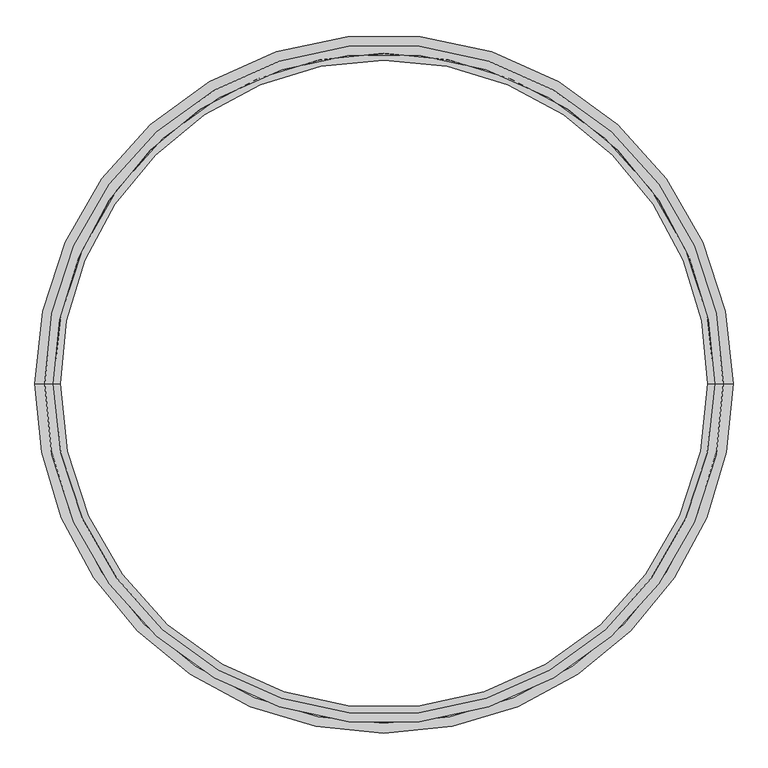
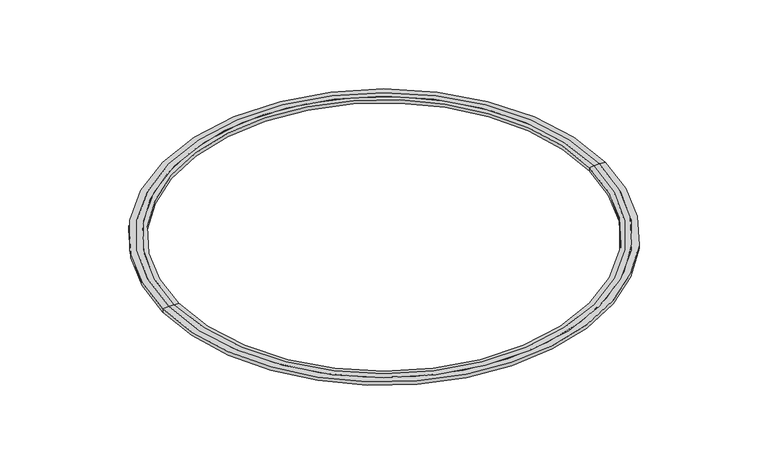
"""IFC4 building model written with IfcOpenShell, lengths in millimetres: proxy geometry, ringbeam_standard : ringbeam_standard."""

from ifc_helpers import new_model, si_unit, frame, origin, place, context, project, spatial, polyline, circle_curve, source, transform, mapped, element, save
from ifc_brep_helpers import plane_surface, cylinder_surface, revolved_surface, advanced_brep


def generic_models_15bcfeb5(model_context):
    return source(origin(), model_context, "Body", "AdvancedBrep", [
        advanced_brep(
        [(10625.0, 0.0, 180.0), (-10625.0, 0.0, 180.0), (-10625.0, 0.0, 0.0), (10625.0, 0.0, 0.0), (10845.0, 0.0, 200.0), (-10845.0, 0.0, 200.0), (11139.2387287, 0.0, 200.0), (-11139.2387287, 0.0, 200.0), (11455.0, 0.0, 180.0), (-11455.0, 0.0, 180.0), (11455.0, 0.0, 0.0), (-11455.0, 0.0, 0.0)],
        [
            (0, 1, circle_curve(frame((0.0, 0.0, 180.0), z_axis=(0.0, 0.0, 1.0), x_axis=(-1.0, 0.0, 0.0)), 10625.0)),
            (1, 2),
            (2, 3, circle_curve(frame((0.0, 0.0, 0.0), z_axis=(0.0, 0.0, -1.0), x_axis=(-1.0, 0.0, 0.0)), 10625.0)),
            (3, 0),
            (1, 0, circle_curve(frame((0.0, 0.0, 180.0), z_axis=(0.0, 0.0, 1.0), x_axis=(-1.0, 0.0, 0.0)), 10625.0)),
            (3, 2, circle_curve(frame((0.0, 0.0, 0.0), z_axis=(0.0, 0.0, -1.0), x_axis=(-1.0, 0.0, 0.0)), 10625.0)),
            (4, 5, circle_curve(frame((0.0, 0.0, 200.0), z_axis=(0.0, 0.0, 1.0), x_axis=(-1.0, 0.0, 0.0)), 10845.0)),
            (5, 1),
            (0, 4),
            (5, 4, circle_curve(frame((0.0, 0.0, 200.0), z_axis=(0.0, 0.0, 1.0), x_axis=(-1.0, 0.0, 0.0)), 10845.0)),
            (6, 7, circle_curve(frame((0.0, 0.0, 200.0), z_axis=(0.0, 0.0, 1.0), x_axis=(-1.0, 0.0, 0.0)), 11139.2387287)),
            (7, 5),
            (4, 6),
            (7, 6, circle_curve(frame((0.0, 0.0, 200.0), z_axis=(0.0, 0.0, 1.0), x_axis=(-1.0, 0.0, 0.0)), 11139.2387287)),
            (8, 9, circle_curve(frame((0.0, 0.0, 180.0), z_axis=(0.0, 0.0, 1.0), x_axis=(-1.0, 0.0, 0.0)), 11455.0)),
            (9, 7),
            (6, 8),
            (9, 8, circle_curve(frame((0.0, 0.0, 180.0), z_axis=(0.0, 0.0, 1.0), x_axis=(-1.0, 0.0, 0.0)), 11455.0)),
            (10, 11, circle_curve(frame((0.0, 0.0, 0.0), z_axis=(0.0, 0.0, 1.0), x_axis=(-1.0, 0.0, 0.0)), 11455.0)),
            (11, 9),
            (8, 10),
            (11, 10, circle_curve(frame((0.0, 0.0, 0.0), z_axis=(0.0, 0.0, 1.0), x_axis=(-1.0, 0.0, 0.0)), 11455.0)),
            (2, 11),
            (10, 3),
        ],
        [
            revolved_surface(polyline([(-10625.0, 0.0, 0.0), (-10625.0, 0.0, 180.0)]), (0.0, 0.0, 2000.0), (0.0, 0.0, -1.0)),
            revolved_surface(polyline([(-10625.0, 0.0, 180.0), (-10845.0, 0.0, 200.0)]), (0.0, 0.0, 2000.0), (0.0, 0.0, -1.0)),
            plane_surface(frame((0.0, 0.0, 200.0), z_axis=(0.0, 0.0, 1.0), x_axis=(-1.0, 0.0, 0.0))),
            revolved_surface(polyline([(-11139.2387287, 0.0, 200.0), (-11455.0, 0.0, 180.0)]), (0.0, 0.0, 2000.0), (0.0, 0.0, -1.0)),
            cylinder_surface(frame((0.0, 0.0, 2000.0), z_axis=(0.0, 0.0, -1.0), x_axis=(-1.0, 0.0, 0.0)), 11455.0),
            plane_surface(frame((0.0, 0.0, 0.0), z_axis=(0.0, 0.0, -1.0), x_axis=(-1.0, 0.0, 0.0))),
        ],
        [
            (0, [[1, 2, 3, 4]]),
            (0, [[5, -4, 6, -2]]),
            (1, [[7, 8, -1, 9]]),
            (1, [[10, -9, -5, -8]]),
            (2, [[11, 12, -7, 13]]),
            (2, [[14, -13, -10, -12]]),
            (3, [[15, 16, -11, 17]]),
            (3, [[18, -17, -14, -16]]),
            (4, [[19, 20, -15, 21]]),
            (4, [[22, -21, -18, -20]]),
            (5, [[-3, 23, -19, 24]]),
            (5, [[-6, -24, -22, -23]]),
        ],
    ),
    ])


if __name__ == "__main__":
    model = new_model("IFC4")
    model_context = context("Model", 3, world=origin())
    ifc_project = project(units=[si_unit("LENGTHUNIT", "METRE", prefix="MILLI")], contexts=[model_context])
    site = spatial("IfcSite", under=ifc_project)
    building = spatial("IfcBuilding", under=site)
    placement = place(None, origin())
    generic_models_shape = generic_models_15bcfeb5(model_context)
    element("IfcBuildingElementProxy", 1, Name="ringbeam_standard : ringbeam_standard", ObjectType="ringbeam_standard : ringbeam_standard", at=placement, inside=building, context=model_context, shape_type="MappedRepresentation", body=[
        mapped(generic_models_shape, transform((0.0, 0.0, 0.0), x_axis=(1.0, 0.0, 0.0), y_axis=(0.0, 1.0, 0.0), z_axis=(0.0, 0.0, 1.0))),
    ])
    save(model, "model.ifc")

# Revit data of these elements
# Project information
#   Company Address = "Fabriksvej 8, V. Lyby DK-7800 Skive"
#   Company E-mail = "info@aconsult.dk"
#   Company Phone = "+45 9687 5800"
#   Company Website = "www.aconsult.dk"
#   Concrete Strength = "CXX/XX"
#   Exposure Class = "XX"
#   Recept = "XX"
#   Kontrolklasse DK = "XX"
#   Panel Supplier = "Example - RC Beton"
#   Company Fax = "+45 9687 5858"
#   Organization Name = "A-CONSULT AGRO A/S"
#   Project Issue Date = "Issue Date"
#   Project Status = "FOR APPROVAL"
#   Client Name = "Client Name"
#   Project Address = "Enter address here"
#   Project Name = "Project Name"
#   Project Number = "XXXXXX"
# Type "ringbeam_standard : ringbeam_standard"
#   R outside [instance default] = 10000 mm
#   R inside [instance default] = 9000 mm
#   Outside Width [instance default] = 220 mm
#   Inside Width [instance default] = 220 mm
#   Default Elevation = 0
# Element 1 (IfcBuildingElementProxy, "ringbeam_standard : ringbeam_standard")
#   R outside = 11455 mm
#   R inside = 10625 mm
#   Outside Width = 315.761 mm
